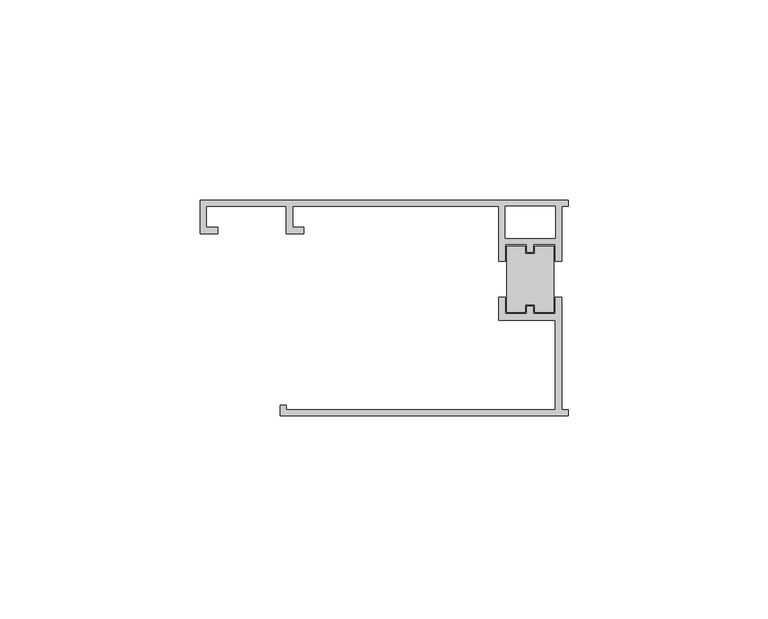
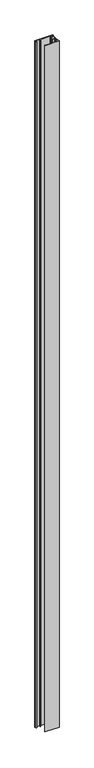
"""IFC4 building model written with IfcOpenShell, lengths in millimetres: proxy geometry, Generic Models 2:Generic Models 2:310765:Generic Models 2:310765 : Generic Models 2:Generic Models 2:310765:59 : Generic Models 2:Generic Models 2:310765:Generic Models 2:310765 : Generic Models 2:Generic Models 2:310765:300385."""

import ifcopenshell
import ifcopenshell.guid

model = None  # the IFC model being written
_history = None  # IfcOwnerHistory: only IFC2X3 demands one
_inside = {}  # id of a spatial element -> (the spatial element, [elements in it])
_under = {}  # id of a project, library or spatial element -> (it, [spatial elements below it])
_declared = {}  # id of a project -> (the project, [libraries it declares])
_typed = {}  # id of a type object -> (the type object, [elements of that type])
_made_of = {}  # id of a material, layer set ... -> (it, [elements and type objects made of it])


def new_model(schema):
    """Start an empty IFC model of exactly this schema.

    Asked for "IFC4X3", IfcOpenShell would pick the latest addendum, in which some entities
    have other attributes; the version numbers below select the first issue.
    IFC2X3 requires an IfcOwnerHistory on every rooted entity: one is made here for all.
    """
    global model, _history
    if schema == "IFC4X3":
        model = ifcopenshell.file(schema_version=(4, 3, 0, 0))
    else:
        model = ifcopenshell.file(schema=schema)
    _inside.clear()
    _under.clear()
    _declared.clear()
    _typed.clear()
    _made_of.clear()
    _history = None
    if model.schema == "IFC2X3":
        org = make("IfcOrganization", Name="unknown")
        user = make(
            "IfcPersonAndOrganization",
            ThePerson=make("IfcPerson", FamilyName="unknown"),
            TheOrganization=org,
        )
        app = make(
            "IfcApplication",
            ApplicationDeveloper=org,
            Version="unknown",
            ApplicationFullName="unknown",
            ApplicationIdentifier="unknown",
        )
        _history = make(
            "IfcOwnerHistory",
            OwningUser=user,
            OwningApplication=app,
            ChangeAction="ADDED",
            CreationDate=0,
        )
    return model


def make(cls, **values):
    """One entity of the class cls with the attributes given. An attribute that is None is left unset."""
    return model.create_entity(
        cls, **{name: value for name, value in values.items() if value is not None}
    )


def rooted(cls, **values):
    """An entity with a GlobalId (a new one), such as an element, a storey or a relation."""
    return make(cls, GlobalId=ifcopenshell.guid.new(), OwnerHistory=_history, **values)


def si_unit(unit_type, name, prefix=None):
    """IfcSIUnit, for example si_unit("LENGTHUNIT", "METRE", prefix="MILLI")."""
    return make("IfcSIUnit", UnitType=unit_type, Prefix=prefix, Name=name)


def assignment(units):
    """IfcUnitAssignment: the units of a project."""
    return None if units is None else make("IfcUnitAssignment", Units=units)


def point(xyz):
    """IfcCartesianPoint."""
    return None if xyz is None else make("IfcCartesianPoint", Coordinates=xyz)


def direction(xyz):
    """IfcDirection."""
    return None if xyz is None else make("IfcDirection", DirectionRatios=xyz)


def frame(location, z_axis=None, x_axis=None):
    """IfcAxis2Placement3D, a coordinate frame: its origin and axes. An axis left out is left unset."""
    return make(
        "IfcAxis2Placement3D",
        Location=point(location),
        Axis=direction(z_axis),
        RefDirection=direction(x_axis),
    )


def origin():
    """The frame at (0, 0, 0) with its axes left unset."""
    return frame((0.0, 0.0, 0.0))


def place(relative_to, where):
    """IfcLocalPlacement: puts the frame where relative to a parent placement (None: the world)."""
    return make(
        "IfcLocalPlacement", PlacementRelTo=relative_to, RelativePlacement=where
    )


def context(
    kind, dimensions, precision=None, world=None, true_north=None, identifier=None
):
    """IfcGeometricRepresentationContext, for example the 3D "Model" context."""
    return make(
        "IfcGeometricRepresentationContext",
        ContextIdentifier=identifier,
        ContextType=kind,
        CoordinateSpaceDimension=dimensions,
        Precision=precision,
        WorldCoordinateSystem=world,
        TrueNorth=true_north,
    )


def project(units=None, contexts=None):
    """IfcProject with its units and contexts."""
    return rooted(
        "IfcProject",
        Name="project",
        RepresentationContexts=contexts,
        UnitsInContext=assignment(units),
    )


def spatial(cls, under=None, at=None, **own):
    """A site, building, storey or space (cls), placed at a placement, below another one or the project."""
    s = rooted(cls, ObjectPlacement=at, **own)
    if under is not None:
        _under.setdefault(under.id(), (under, []))[1].append(s)
    return s


def polyline(points):
    """IfcPolyline through the points."""
    return make("IfcPolyline", Points=[point(p) for p in points])


def outline(outer, holes=None, kind="AREA"):
    """IfcArbitraryClosedProfileDef: a profile drawn as a closed curve; with holes, ...WithVoids."""
    if holes is None:
        return make("IfcArbitraryClosedProfileDef", ProfileType=kind, OuterCurve=outer)
    return make(
        "IfcArbitraryProfileDefWithVoids",
        ProfileType=kind,
        OuterCurve=outer,
        InnerCurves=holes,
    )


def extrude(swept, where, along, depth):
    """IfcExtrudedAreaSolid: the profile swept, set in the frame where, extruded along a direction by depth."""
    return make(
        "IfcExtrudedAreaSolid",
        SweptArea=swept,
        Position=where,
        ExtrudedDirection=direction(along),
        Depth=depth,
    )


def shape(context_of_items, identifier, shape_type, items):
    """IfcShapeRepresentation: the items that make up one representation, for example the "Body"."""
    return make(
        "IfcShapeRepresentation",
        ContextOfItems=context_of_items,
        RepresentationIdentifier=identifier,
        RepresentationType=shape_type,
        Items=items,
    )


def source(mapping_origin, context_of_items, identifier, shape_type, items):
    """IfcRepresentationMap: a shape defined once, which mapped items show again and again."""
    return make(
        "IfcRepresentationMap",
        MappingOrigin=mapping_origin,
        MappedRepresentation=shape(context_of_items, identifier, shape_type, items),
    )


def transform(
    local_origin,
    x_axis=None,
    y_axis=None,
    z_axis=None,
    scale=None,
    scale2=None,
    scale3=None,
    uniform=True,
):
    """IfcCartesianTransformationOperator3D, or its non-uniform kind. x_axis, y_axis, z_axis: its Axis1, 2, 3."""
    if uniform:
        return make(
            "IfcCartesianTransformationOperator3D",
            Axis1=direction(x_axis),
            Axis2=direction(y_axis),
            LocalOrigin=point(local_origin),
            Scale=scale,
            Axis3=direction(z_axis),
        )
    return make(
        "IfcCartesianTransformationOperator3DnonUniform",
        Axis1=direction(x_axis),
        Axis2=direction(y_axis),
        LocalOrigin=point(local_origin),
        Scale=scale,
        Axis3=direction(z_axis),
        Scale2=scale2,
        Scale3=scale3,
    )


def mapped(mapping_source, mapping_target):
    """IfcMappedItem: shows the shape of a source again, moved by a transform."""
    return make(
        "IfcMappedItem", MappingSource=mapping_source, MappingTarget=mapping_target
    )


def made_of(thing, what):
    """Note that an element or type object is made of a material, layer set ...; save() writes the relation."""
    if what is not None:
        _made_of.setdefault(what.id(), (what, []))[1].append(thing)
    return thing


def element(
    cls,
    number,
    at=None,
    inside=None,
    cuts=None,
    type_object=None,
    material=None,
    context=None,
    identifier="Body",
    shape_type=None,
    held_by="IfcProductDefinitionShape",
    body=None,
    shapes=None,
    **own,
):
    """One element of the class cls, such as IfcWall. Its Tag is "e" and its number.

    at: its placement. inside: the storey or other place that contains it. cuts: it is an
    opening in that element (IfcRelVoidsElement). A single representation is given by context,
    identifier, shape_type and body (its items); several are given by shapes. held_by: the class
    of the entity that holds the representations. save() writes the other relations.
    """
    e = rooted(cls, Tag="e%d" % number, ObjectPlacement=at, **own)
    if body is not None:
        shapes = [shape(context, identifier, shape_type, body)]
    if shapes is not None:
        e.Representation = make(held_by, Representations=shapes)
    if inside is not None:
        _inside.setdefault(inside.id(), (inside, []))[1].append(e)
    if cuts is not None:
        rooted(
            "IfcRelVoidsElement", RelatingBuildingElement=cuts, RelatedOpeningElement=e
        )
    if type_object is not None:
        _typed.setdefault(type_object.id(), (type_object, []))[1].append(e)
    return made_of(e, material)


def aggregate(whole, parts):
    """IfcRelAggregates: a whole, such as a stair, and the parts it consists of."""
    return rooted("IfcRelAggregates", RelatingObject=whole, RelatedObjects=parts)


def save(model, path):
    """Write the relations noted so far, then the file.

    IfcRelAggregates (storeys below a building ...), IfcRelContainedInSpatialStructure (elements
    in a storey), IfcRelDefinesByType, IfcRelAssociatesMaterial and IfcRelDeclares: one each for
    every whole, place, type object, material and project.
    """
    for whole, parts in _under.values():
        aggregate(whole, parts)
    for where, things in _inside.values():
        rooted(
            "IfcRelContainedInSpatialStructure",
            RelatedElements=things,
            RelatingStructure=where,
        )
    for kind, things in _typed.values():
        rooted("IfcRelDefinesByType", RelatedObjects=things, RelatingType=kind)
    for what, things in _made_of.values():
        rooted("IfcRelAssociatesMaterial", RelatedObjects=things, RelatingMaterial=what)
    for by, libraries in _declared.values():
        rooted("IfcRelDeclares", RelatingContext=by, RelatedDefinitions=libraries)
    model.write(path)


def generic_models_5ed1a8d4(model_context):
    return source(origin(), model_context, "Body", "SweptSolid", [
        extrude(outline(polyline([(564983.3960122, -568246.416762), (564983.3960122, -568229.8645058), (564988.0935108, -568229.8645058), (564988.0935108, -568231.7899212), (564990.4747608, -568231.7899212), (564990.4747608, -568229.8645058), (564995.1722595, -568229.8645058), (564995.1722595, -568246.416762), (564990.4747608, -568246.416762), (564990.4747608, -568244.4913465), (564988.0935108, -568244.4913465), (564988.0935108, -568246.416762), (564983.3960122, -568246.416762)])), frame((0.0, 0.0, 4860.0679991), z_axis=(0.0, 0.0, 1.0), x_axis=(1.0, 0.0, 0.0)), (0.0, 0.0, 1.0), 3695.7),
        extrude(outline(polyline([(564906.7441345, -568226.7958673), (564906.7441345, -568218.3494958), (564998.7441345, -568218.3494958), (564998.7441345, -568219.9369958), (564997.1566345, -568219.9369958), (564997.1566345, -568233.6348183), (564995.5691345, -568233.6348183), (564995.5691345, -568229.4676308), (564990.0778858, -568229.4676308), (564990.0778858, -568231.3930462), (564988.4903858, -568231.3930462), (564988.4903858, -568229.4676308), (564982.9991372, -568229.4676308), (564982.9991372, -568233.6348183), (564981.4116372, -568233.6348183), (564981.4116372, -568219.9369958), (564929.9191345, -568219.9369958), (564929.9191345, -568225.2083673), (564932.718961, -568225.2083673), (564932.718961, -568226.7958673), (564928.3316345, -568226.7958673), (564928.3316345, -568219.9369958), (564908.3316345, -568219.9369958), (564908.3316345, -568225.2083673), (564911.131461, -568225.2083673), (564911.131461, -568226.7958673), (564906.7441345, -568226.7958673)]), holes=[polyline([(564982.9991372, -568219.9369958), (564982.9991372, -568227.8801308), (564995.5691345, -568227.8801308), (564995.5691345, -568219.9369958), (564982.9991372, -568219.9369958)])]), frame((0.0, 0.0, 4860.0679991), z_axis=(0.0, 0.0, 1.0), x_axis=(1.0, 0.0, 0.0)), (0.0, 0.0, 1.0), 3695.7),
        extrude(outline(polyline([(564998.7441345, -568270.7619958), (564998.7441345, -568272.3494958), (564926.7441345, -568272.3494958), (564926.7441345, -568269.6344059), (564928.3316345, -568269.6344059), (564928.3316345, -568270.7619958), (564995.5691345, -568270.7619958), (564995.5691345, -568248.401137), (564981.4116372, -568248.401137), (564981.4116372, -568242.6464495), (564982.9991372, -568242.6464495), (564982.9991372, -568246.813637), (564988.4903858, -568246.813637), (564988.4903858, -568244.8882215), (564990.0778858, -568244.8882215), (564990.0778858, -568246.813637), (564995.5691345, -568246.813637), (564995.5691345, -568242.6464495), (564997.1566345, -568242.6464495), (564997.1566345, -568270.7619958), (564998.7441345, -568270.7619958)])), frame((0.0, 0.0, 4860.0679991), z_axis=(0.0, 0.0, 1.0), x_axis=(1.0, 0.0, 0.0)), (0.0, 0.0, 1.0), 3695.7),
    ])


if __name__ == "__main__":
    model = new_model("IFC4")
    model_context = context("Model", 3, world=origin())
    ifc_project = project(units=[si_unit("LENGTHUNIT", "METRE", prefix="MILLI")], contexts=[model_context])
    site = spatial("IfcSite", under=ifc_project)
    building = spatial("IfcBuilding", under=site)
    placement = place(None, origin())
    generic_models_shape = generic_models_5ed1a8d4(model_context)
    element("IfcBuildingElementProxy", 1, Name="Generic Models 2:Generic Models 2:310765:Generic Models 2:310765 : Generic Models 2:Generic Models 2:310765:59 : Generic Models 2:Generic Models 2:310765:Generic Models 2:310765 : Generic Models 2:Generic Models 2:310765:300385", ObjectType="Generic Models 2:Generic Models 2:310765:Generic Models 2:310765 : Generic Models 2:Generic Models 2:310765:59 : Generic Models 2:Generic Models 2:310765:Generic Models 2:310765 : Generic Models 2:Generic Models 2:310765:300385", at=placement, inside=building, context=model_context, shape_type="MappedRepresentation", body=[
        mapped(generic_models_shape, transform((0.0, 0.0, 0.0), x_axis=(1.0, 0.0, 0.0), y_axis=(0.0, 1.0, 0.0), z_axis=(0.0, 0.0, 1.0))),
    ])
    save(model, "model.ifc")

# Revit data of these elements
# Type "Generic Models 2:Generic Models 2:310765:Generic Models 2:310765 : Generic Models 2:Generic Models 2:310765:59 : Generic Models 2:Generic Models 2:310765:Generic Models 2:310765 : Generic Models 2:Generic Models 2:310765:300385"
#   NameOverride = "Generic Models 2:Generic Models 2:310765:Generic Models 2:310765 : Generic Models 2:Generic Models 2:310765:300385"
#   ObjectTypeOverride = "Generic Models 2:310765 : Generic Models 2:Generic Models 2:310765"
#   Reference = "Generic Models 2"
#   Tag = "300385"
# Element 1 (IfcBuildingElementProxy, "Generic Models 2:Generic Models 2:310765:Generic Models 2:310765 : Generic Models 2:Generic Models 2:310765:59 : Generic Models 2:Generic Models 2:310765:Generic Models 2:310765 : Generic Models 2:Generic Models 2:310765:300385")
#   Materials on its faces: "THERMAL BROKEN ALUMINUM STOREFRONT FOR POLYCARBONATE"
# Materials
#   "THERMAL BROKEN ALUMINUM STOREFRONT FOR POLYCARBONATE": class "Unassigned", colour RGB 244 244 244, transparency 0, Keynote = "M07611300.01", Cost = 0
